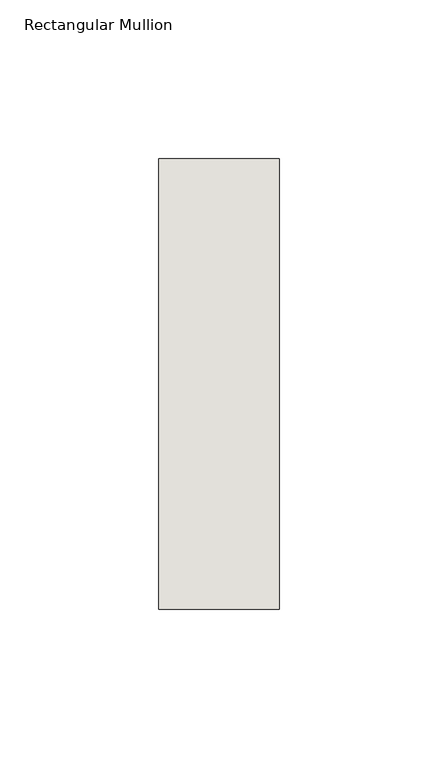
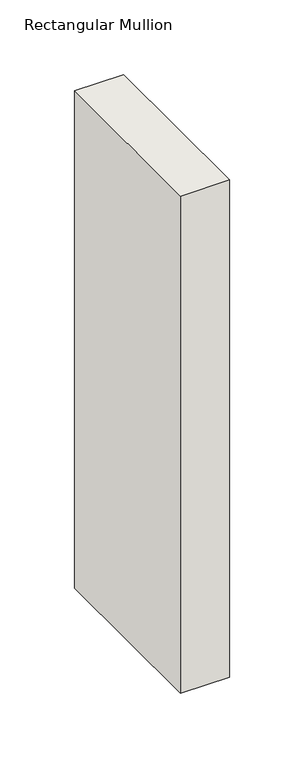
"""IFC4 building model written with IfcOpenShell, lengths in millimetres: wall geometry, Rectangular Mullion : NLRS_21_CWM_hsb-regel 38x142_gen_rsf."""

from ifc_helpers import new_model, si_unit, frame, origin, place, context, project, spatial, polyline, outline, extrude, source, transform, mapped, element, save


def rectangular_mullion_2a836202(model_context):
    return source(origin(), model_context, "Body", "SweptSolid", [
        extrude(outline(polyline([(0.0, -71.0), (-38.0, -71.0), (-38.0, 71.0), (0.0, 71.0), (0.0, -71.0)])), frame((0.0, 0.0, -407.0000003), z_axis=(0.0, 0.0, 1.0), x_axis=(1.0, 0.0, 0.0)), (0.0, 0.0, 1.0), 407.0000003),
    ])


if __name__ == "__main__":
    model = new_model("IFC4")
    model_context = context("Model", 3, world=origin())
    ifc_project = project(units=[si_unit("LENGTHUNIT", "METRE", prefix="MILLI")], contexts=[model_context])
    site = spatial("IfcSite", under=ifc_project)
    building = spatial("IfcBuilding", under=site)
    placement = place(None, origin())
    rectangular_mullion_shape = rectangular_mullion_2a836202(model_context)
    element("IfcWall", 1, ObjectType="Rectangular Mullion : NLRS_21_CWM_hsb-regel 38x142_gen_rsf", at=placement, inside=building, context=model_context, shape_type="MappedRepresentation", body=[
        mapped(rectangular_mullion_shape, transform((0.0, 0.0, 0.0), x_axis=(1.0, 0.0, 0.0), y_axis=(0.0, 1.0, 0.0), z_axis=(0.0, 0.0, 1.0))),
    ])
    save(model, "model.ifc")

# Revit data of these elements
# Type "Rectangular Mullion : NLRS_21_CWM_hsb-regel 38x142_gen_rsf"
#   Type IfcGUID = "07M7mRoiH1CR8m_RSKIwpF"
#   Assembly Code = "21.10"
#   IfcExportAs = "IfcWall"
#   built-in parameter 1007322 = 0.465879 (stored number, unit not read)
#   built-in parameter 1007321 = 0.062336 (stored number, unit not read)
#   built-in parameter 1007320 = 0.062336 (stored number, unit not read)
# Element 1 (IfcWall, "Rectangular Mullion : NLRS_21_CWM_hsb-regel 38x142_gen_rsf")
#   Materials on its faces: "NLRS_i2_hout naaldhout vuren_gen_rsf"
# Materials
#   "NLRS_i2_hout naaldhout vuren_gen_rsf": class "I - Hout", colour RGB 234 199 147, transparency 0, Keynote = "i2", Manufacturer = "Revit Standards Foundation", URL = "www.revitstandards.org", Description = "hout vuren", Cost = 0
